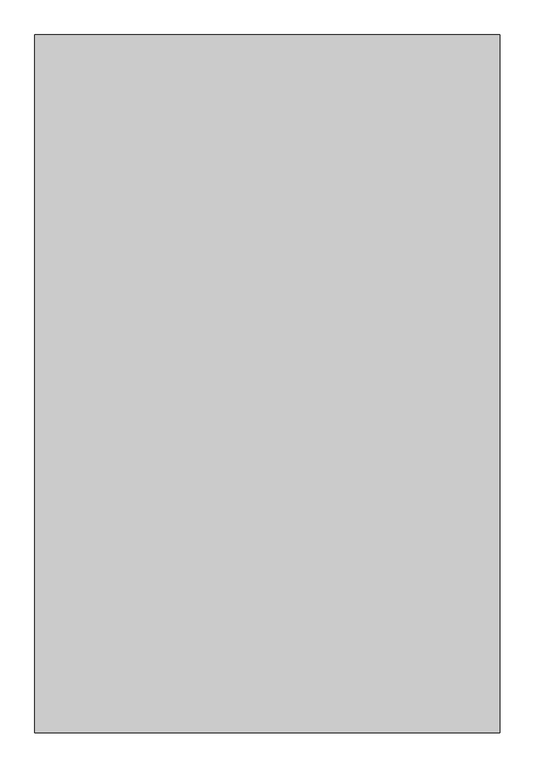
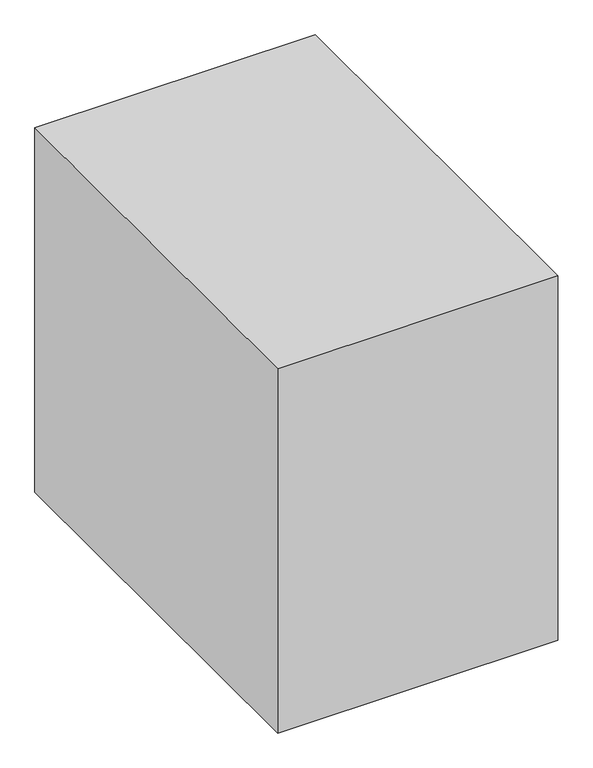
"""IFC4 building model written with IfcOpenShell, lengths in millimetres: proxy geometry, Space Planning Box_hec : Space Planning Box_hec."""

from ifc_helpers import new_model, si_unit, origin, origin_with_axes, place, context, project, spatial, polyline, outline, extrude, source, transform, mapped, element, save


def generic_models_cc1dae17(model_context):
    return source(origin(), model_context, "Body", "SweptSolid", [
        extrude(outline(polyline([(2000.0, 3000.0), (2000.0, -3000.0), (-2000.0, -3000.0), (-2000.0, 3000.0), (2000.0, 3000.0)])), origin_with_axes(), (0.0, 0.0, 1.0), 5500.0),
    ])


if __name__ == "__main__":
    model = new_model("IFC4")
    model_context = context("Model", 3, world=origin())
    ifc_project = project(units=[si_unit("LENGTHUNIT", "METRE", prefix="MILLI")], contexts=[model_context])
    site = spatial("IfcSite", under=ifc_project)
    building = spatial("IfcBuilding", under=site)
    placement = place(None, origin())
    generic_models_shape = generic_models_cc1dae17(model_context)
    element("IfcBuildingElementProxy", 1, Name="Space Planning Box_hec : Space Planning Box_hec", ObjectType="Space Planning Box_hec : Space Planning Box_hec", at=placement, inside=building, context=model_context, shape_type="MappedRepresentation", body=[
        mapped(generic_models_shape, transform((0.0, 0.0, 0.0), x_axis=(1.0, 0.0, 0.0), y_axis=(0.0, 1.0, 0.0), z_axis=(0.0, 0.0, 1.0))),
    ])
    save(model, "model.ifc")

# Revit data of these elements
# Type "Space Planning Box_hec : Space Planning Box_hec"
#   Type Comments = "..."
#   Room Name [instance default] = "?"
#   Interior Finish [instance default] = ""
#   Exterior Finish [instance default] = ""
#   Department [instance default] = ""
#   Assembly Code = "..."
#   ceiling height [instance default] = 0
#   Width [instance default] = 1524 mm
#   Program Area [instance default] = 0.00 m²
#   Length [instance default] = 1524 mm
#   Height [instance default] = 1524 mm
#   Area [instance default] = 2.32258 m²
#   Fill Color [instance default] = Cyan
#   Default Elevation = 0
# Element 1 (IfcBuildingElementProxy, "Space Planning Box_hec : Space Planning Box_hec")
#   Room Name = "Staircase"
#   Exterior Finish = "N/A..N/A,,EW2..N/A..N/A"
#   Department = "PATHV1"
#   Width = 4000 mm
#   Program Area = 24.00 m²
#   Length = 6000 mm
#   Height = 5500 mm
#   Area = 24.00 m²
#   Fill Color = Green
#   Materials on its faces: "Green"
# Materials
#   "Cyan": class "Generic", colour RGB 0 255 255, transparency 0.2, Cost = 0
#   "Green": class "Generic", colour RGB 0 128 0, transparency 0.2, Cost = 0
